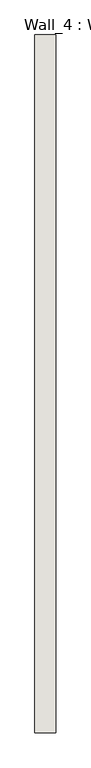
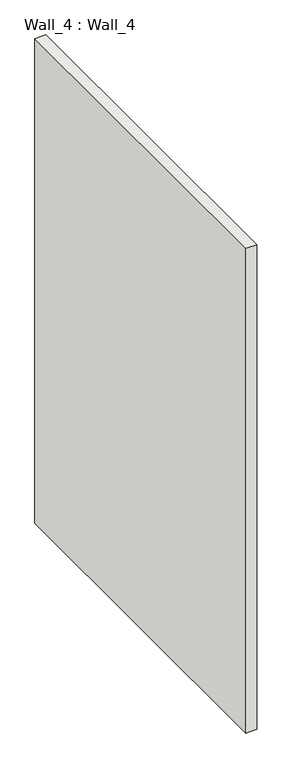
"""IFC4 building model written with IfcOpenShell, lengths in millimetres: wall geometry, Wall_4 : Wall_4."""

from ifc_helpers import new_model, si_unit, origin, origin_with_axes, place, context, project, spatial, polyline, outline, extrude, source, transform, mapped, element, save


def wall_4_wall_4_e46e00ff(model_context):
    return source(origin(), model_context, "Body", "SweptSolid", [
        extrude(outline(polyline([(100.0, 15700.0), (100.0, 12350.0), (0.0, 12350.0), (0.0, 15700.0), (100.0, 15700.0)])), origin_with_axes(), (0.0, 0.0, 1.0), 4700.0),
    ])


if __name__ == "__main__":
    model = new_model("IFC4")
    model_context = context("Model", 3, world=origin())
    ifc_project = project(units=[si_unit("LENGTHUNIT", "METRE", prefix="MILLI")], contexts=[model_context])
    site = spatial("IfcSite", under=ifc_project)
    building = spatial("IfcBuilding", under=site)
    placement = place(None, origin())
    wall_4_wall_4_shape = wall_4_wall_4_e46e00ff(model_context)
    element("IfcWall", 1, ObjectType="Wall_4 : Wall_4", at=placement, inside=building, context=model_context, shape_type="MappedRepresentation", body=[
        mapped(wall_4_wall_4_shape, transform((0.0, 0.0, 0.0), x_axis=(1.0, 0.0, 0.0), y_axis=(0.0, 1.0, 0.0), z_axis=(0.0, 0.0, 1.0))),
    ])
    save(model, "model.ifc")

# Revit data of these elements
# Type "Wall_4 : Wall_4"
#   NameOverride = "Wall_4"
# Element 1 (IfcWall, "Wall_4 : Wall_4")
#   Materials on its faces: "IfcSurfaceStyle #33"
# Materials
#   "IfcSurfaceStyle #33": class "Unassigned", colour RGB 214 214 214, transparency 0
